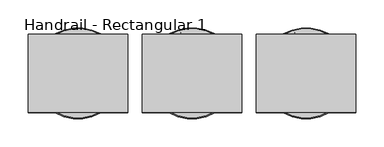
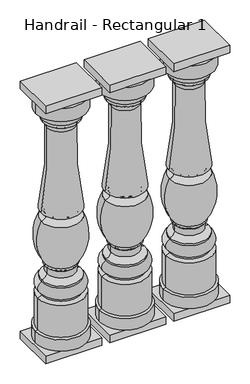
"""IFC4 building model written with IfcOpenShell, lengths in millimetres: railing geometry, Handrail - Rectangular 1."""

from ifc_helpers import new_model, si_unit, point, frame, origin, place, context, project, spatial, polyline, circle_curve, ellipse_curve, trimmed, outline, extrude, source, transform, mapped, element, save
from ifc_brep_helpers import plane_surface, cylinder_surface, revolved_surface, advanced_brep


def handrail_rectangular_1_f9308160(model_context):
    return source(origin(), model_context, "Body", "SolidModel", [
        advanced_brep(
        [(7223.6521895, -1665.6164768, 939.8), (7144.2771895, -1665.6164768, 939.8), (7303.0271895, -1665.6164768, 939.8), (7304.6146895, -1665.6164768, 127.0), (7142.6896895, -1665.6164768, 127.0), (7223.6521895, -1665.6164768, 127.0), (7304.6146895, -1665.6164768, 165.2785542), (7142.6896895, -1665.6164768, 165.2785542), (7297.4709395, -1665.6164768, 168.275), (7149.8334395, -1665.6164768, 168.275), (7297.4709395, -1665.6164768, 274.7335284), (7149.8334395, -1665.6164768, 274.7335284), (7284.7709395, -1665.6164768, 280.19375), (7162.5334395, -1665.6164768, 280.19375), (7284.7709395, -1665.6164768, 286.54375), (7162.5334395, -1665.6164768, 286.54375), (7284.7709395, -1665.6164768, 324.64375), (7162.5334395, -1665.6164768, 324.64375), (7284.7709395, -1665.6164768, 330.99375), (7162.5334395, -1665.6164768, 330.99375), (7269.0640435, -1665.6164768, 347.276159), (7178.2403356, -1665.6164768, 347.276159), (7269.0640435, -1665.6164768, 368.8906259), (7178.2403356, -1665.6164768, 368.8906259), (7273.6584395, -1665.6164768, 373.85625), (7173.6459395, -1665.6164768, 373.85625), (7273.6584395, -1665.6164768, 381.4842759), (7173.6459395, -1665.6164768, 381.4842759), (7286.3584395, -1665.6164768, 527.84375), (7160.9459395, -1665.6164768, 527.84375), (7286.3584395, -1665.6164768, 556.41875), (7160.9459395, -1665.6164768, 556.41875), (7267.8243377, -1665.6164768, 836.1713606), (7179.4800414, -1665.6164768, 836.1713606), (7280.8021895, -1665.6164768, 858.04375), (7166.5021895, -1665.6164768, 858.04375), (7280.8021895, -1665.6164768, 866.775), (7166.5021895, -1665.6164768, 866.775), (7291.9146895, -1665.6164768, 892.175), (7155.3896895, -1665.6164768, 892.175), (7303.0271895, -1665.6164768, 895.35), (7144.2771895, -1665.6164768, 895.35)],
        [
            (0, 1),
            (1, 2, circle_curve(frame((7223.6521895, -1665.6164768, 939.8), z_axis=(0.0, 0.0, 1.0), x_axis=(-1.0, 0.0, 0.0)), 79.375)),
            (2, 0),
            (2, 1, circle_curve(frame((7223.6521895, -1665.6164768, 939.8), z_axis=(0.0, 0.0, 1.0), x_axis=(-1.0, 0.0, 0.0)), 79.375)),
            (3, 4, circle_curve(frame((7223.6521895, -1665.6164768, 127.0), z_axis=(0.0, 0.0, -1.0), x_axis=(-1.0, 0.0, 0.0)), 80.9625)),
            (4, 5),
            (5, 3),
            (4, 3, circle_curve(frame((7223.6521895, -1665.6164768, 127.0), z_axis=(0.0, 0.0, -1.0), x_axis=(-1.0, 0.0, 0.0)), 80.9625)),
            (6, 7, circle_curve(frame((7223.6521895, -1665.6164768, 165.2785542), z_axis=(0.0, 0.0, -1.0), x_axis=(-1.0, 0.0, 0.0)), 80.9625)),
            (7, 4),
            (3, 6),
            (7, 6, circle_curve(frame((7223.6521895, -1665.6164768, 165.2785542), z_axis=(0.0, 0.0, -1.0), x_axis=(-1.0, 0.0, 0.0)), 80.9625)),
            (8, 9, circle_curve(frame((7223.6521895, -1665.6164768, 168.275), z_axis=(0.0, 0.0, -1.0), x_axis=(-1.0, 0.0, 0.0)), 73.81875)),
            (9, 7),
            (6, 8),
            (9, 8, circle_curve(frame((7223.6521895, -1665.6164768, 168.275), z_axis=(0.0, 0.0, -1.0), x_axis=(-1.0, 0.0, 0.0)), 73.81875)),
            (10, 11, circle_curve(frame((7223.6521895, -1665.6164768, 274.7335284), z_axis=(0.0, 0.0, -1.0), x_axis=(-1.0, 0.0, 0.0)), 73.81875)),
            (11, 9),
            (8, 10),
            (11, 10, circle_curve(frame((7223.6521895, -1665.6164768, 274.7335284), z_axis=(0.0, 0.0, -1.0), x_axis=(-1.0, 0.0, 0.0)), 73.81875)),
            (12, 13, circle_curve(frame((7223.6521895, -1665.6164768, 280.19375), z_axis=(0.0, 0.0, -1.0), x_axis=(-1.0, 0.0, 0.0)), 61.11875)),
            (13, 11),
            (10, 12),
            (13, 12, circle_curve(frame((7223.6521895, -1665.6164768, 280.19375), z_axis=(0.0, 0.0, -1.0), x_axis=(-1.0, 0.0, 0.0)), 61.11875)),
            (14, 15, circle_curve(frame((7223.6521895, -1665.6164768, 286.54375), z_axis=(0.0, 0.0, -1.0), x_axis=(-1.0, 0.0, 0.0)), 61.11875)),
            (15, 13),
            (12, 14),
            (15, 14, circle_curve(frame((7223.6521895, -1665.6164768, 286.54375), z_axis=(0.0, 0.0, -1.0), x_axis=(-1.0, 0.0, 0.0)), 61.11875)),
            (16, 17, circle_curve(frame((7223.6521895, -1665.6164768, 324.64375), z_axis=(0.0, 0.0, -1.0), x_axis=(-1.0, 0.0, 0.0)), 61.11875)),
            (17, 15, circle_curve(frame((7170.7987498, -1665.6164768, 305.59375), z_axis=(0.0, -1.0, 0.0), x_axis=(1.0, 0.0, 0.0)), 20.7657856)),
            (14, 16, circle_curve(frame((7276.5056293, -1665.6164768, 305.59375), z_axis=(0.0, -1.0, 0.0), x_axis=(-1.0, 0.0, 0.0)), 20.7657856)),
            (17, 16, circle_curve(frame((7223.6521895, -1665.6164768, 324.64375), z_axis=(0.0, 0.0, -1.0), x_axis=(-1.0, 0.0, 0.0)), 61.11875)),
            (18, 19, circle_curve(frame((7223.6521895, -1665.6164768, 330.99375), z_axis=(0.0, 0.0, -1.0), x_axis=(-1.0, 0.0, 0.0)), 61.11875)),
            (19, 17),
            (16, 18),
            (19, 18, circle_curve(frame((7223.6521895, -1665.6164768, 330.99375), z_axis=(0.0, 0.0, -1.0), x_axis=(-1.0, 0.0, 0.0)), 61.11875)),
            (20, 21, circle_curve(frame((7223.6521895, -1665.6164768, 347.276159), z_axis=(0.0, 0.0, -1.0), x_axis=(-1.0, 0.0, 0.0)), 45.4118539)),
            (21, 19, circle_curve(frame((7163.0004121, -1665.6164768, 346.26035), z_axis=(0.0, 1.0, 0.0), x_axis=(1.0, 0.0, 0.0)), 15.2737402)),
            (18, 20, circle_curve(frame((7284.303967, -1665.6164768, 346.26035), z_axis=(0.0, 1.0, 0.0), x_axis=(-1.0, 0.0, 0.0)), 15.2737402)),
            (21, 20, circle_curve(frame((7223.6521895, -1665.6164768, 347.276159), z_axis=(0.0, 0.0, -1.0), x_axis=(-1.0, 0.0, 0.0)), 45.4118539)),
            (22, 23, circle_curve(frame((7223.6521895, -1665.6164768, 368.8906259), z_axis=(0.0, 0.0, -1.0), x_axis=(-1.0, 0.0, 0.0)), 45.4118539)),
            (23, 21),
            (20, 22),
            (23, 22, circle_curve(frame((7223.6521895, -1665.6164768, 368.8906259), z_axis=(0.0, 0.0, -1.0), x_axis=(-1.0, 0.0, 0.0)), 45.4118539)),
            (24, 25, circle_curve(frame((7223.6521895, -1665.6164768, 373.85625), z_axis=(0.0, 0.0, -1.0), x_axis=(-1.0, 0.0, 0.0)), 50.00625)),
            (25, 23, circle_curve(frame((7173.3940931, -1665.6164768, 369.014959), z_axis=(0.0, 1.0, 0.0), x_axis=(1.0, 0.0, 0.0)), 4.8478372)),
            (22, 24, circle_curve(frame((7273.910286, -1665.6164768, 369.014959), z_axis=(0.0, 1.0, 0.0), x_axis=(-1.0, 0.0, 0.0)), 4.8478372)),
            (25, 24, circle_curve(frame((7223.6521895, -1665.6164768, 373.85625), z_axis=(0.0, 0.0, -1.0), x_axis=(-1.0, 0.0, 0.0)), 50.00625)),
            (26, 27, circle_curve(frame((7223.6521895, -1665.6164768, 381.4842759), z_axis=(0.0, 0.0, -1.0), x_axis=(-1.0, 0.0, 0.0)), 50.00625)),
            (27, 25),
            (24, 26),
            (27, 26, circle_curve(frame((7223.6521895, -1665.6164768, 381.4842759), z_axis=(0.0, 0.0, -1.0), x_axis=(-1.0, 0.0, 0.0)), 50.00625)),
            (28, 29, circle_curve(frame((7223.6521895, -1665.6164768, 527.84375), z_axis=(0.0, 0.0, -1.0), x_axis=(-1.0, 0.0, 0.0)), 62.70625)),
            (29, 27, circle_curve(frame((7291.2829206, -1665.6164768, 465.4226923), z_axis=(0.0, -1.0, 0.0), x_axis=(1.0, 0.0, 0.0)), 144.5133802)),
            (26, 28, circle_curve(frame((7156.0214585, -1665.6164768, 465.4226923), z_axis=(0.0, -1.0, 0.0), x_axis=(-1.0, 0.0, 0.0)), 144.5133802)),
            (29, 28, circle_curve(frame((7223.6521895, -1665.6164768, 527.84375), z_axis=(0.0, 0.0, -1.0), x_axis=(-1.0, 0.0, 0.0)), 62.70625)),
            (30, 31, circle_curve(frame((7223.6521895, -1665.6164768, 556.41875), z_axis=(0.0, 0.0, -1.0), x_axis=(-1.0, 0.0, 0.0)), 62.70625)),
            (31, 29, circle_curve(frame((7161.7940628, -1665.6164768, 542.13125), z_axis=(0.0, 1.0, 0.0), x_axis=(1.0, 0.0, 0.0)), 14.3126507)),
            (28, 30, circle_curve(frame((7285.5103163, -1665.6164768, 542.13125), z_axis=(0.0, 1.0, 0.0), x_axis=(-1.0, 0.0, 0.0)), 14.3126507)),
            (31, 30, circle_curve(frame((7223.6521895, -1665.6164768, 556.41875), z_axis=(0.0, 0.0, -1.0), x_axis=(-1.0, 0.0, 0.0)), 62.70625)),
            (32, 33, circle_curve(frame((7223.6521895, -1665.6164768, 836.1713606), z_axis=(0.0, 0.0, -1.0), x_axis=(-1.0, 0.0, 0.0)), 44.1721482)),
            (33, 31, circle_curve(frame((6049.660691, -1665.6164768, 770.5336134), z_axis=(0.0, 1.0, 0.0), x_axis=(1.0, 0.0, 0.0)), 1131.7243827)),
            (30, 32, circle_curve(frame((8397.6436881, -1665.6164768, 770.5336134), z_axis=(0.0, 1.0, 0.0), x_axis=(-1.0, 0.0, 0.0)), 1131.7243827)),
            (33, 32, circle_curve(frame((7223.6521895, -1665.6164768, 836.1713606), z_axis=(0.0, 0.0, -1.0), x_axis=(-1.0, 0.0, 0.0)), 44.1721482)),
            (34, 35, circle_curve(frame((7223.6521895, -1665.6164768, 858.04375), z_axis=(0.0, 0.0, -1.0), x_axis=(-1.0, 0.0, 0.0)), 57.15)),
            (35, 33, circle_curve(frame((7158.4577367, -1665.6164768, 838.4842616), z_axis=(0.0, 1.0, 0.0), x_axis=(1.0, 0.0, 0.0)), 21.1491562)),
            (32, 34, circle_curve(frame((7288.8466424, -1665.6164768, 838.4842616), z_axis=(0.0, 1.0, 0.0), x_axis=(-1.0, 0.0, 0.0)), 21.1491562)),
            (35, 34, circle_curve(frame((7223.6521895, -1665.6164768, 858.04375), z_axis=(0.0, 0.0, -1.0), x_axis=(-1.0, 0.0, 0.0)), 57.15)),
            (36, 37, circle_curve(frame((7223.6521895, -1665.6164768, 866.775), z_axis=(0.0, 0.0, -1.0), x_axis=(-1.0, 0.0, 0.0)), 57.15)),
            (37, 35),
            (34, 36),
            (37, 36, circle_curve(frame((7223.6521895, -1665.6164768, 866.775), z_axis=(0.0, 0.0, -1.0), x_axis=(-1.0, 0.0, 0.0)), 57.15)),
            (38, 39, circle_curve(frame((7223.6521895, -1665.6164768, 892.175), z_axis=(0.0, 0.0, -1.0), x_axis=(-1.0, 0.0, 0.0)), 68.2625)),
            (39, 37, circle_curve(frame((7184.7272944, -1665.6164768, 889.8793427), z_axis=(0.0, -1.0, 0.0), x_axis=(1.0, 0.0, 0.0)), 29.4272849)),
            (36, 38, circle_curve(frame((7262.5770847, -1665.6164768, 889.8793427), z_axis=(0.0, -1.0, 0.0), x_axis=(-1.0, 0.0, 0.0)), 29.4272849)),
            (39, 38, circle_curve(frame((7223.6521895, -1665.6164768, 892.175), z_axis=(0.0, 0.0, -1.0), x_axis=(-1.0, 0.0, 0.0)), 68.2625)),
            (40, 41, circle_curve(frame((7223.6521895, -1665.6164768, 895.35), z_axis=(0.0, 0.0, -1.0), x_axis=(-1.0, 0.0, 0.0)), 79.375)),
            (41, 39),
            (38, 40),
            (41, 40, circle_curve(frame((7223.6521895, -1665.6164768, 895.35), z_axis=(0.0, 0.0, -1.0), x_axis=(-1.0, 0.0, 0.0)), 79.375)),
            (1, 41),
            (40, 2),
        ],
        [
            plane_surface(frame((7223.6521895, -1665.6164768, 939.8), z_axis=(0.0, 0.0, 1.0), x_axis=(-1.0, 0.0, 0.0))),
            plane_surface(frame((7223.6521895, -1665.6164768, 127.0), z_axis=(0.0, 0.0, -1.0), x_axis=(-1.0, 0.0, 0.0))),
            cylinder_surface(frame((7223.6521895, -1665.6164768, 1009.65), z_axis=(0.0, 0.0, 1.0), x_axis=(-1.0, 0.0, 0.0)), 80.9625),
            revolved_surface(polyline([(7142.6896895, -1665.6164768, 165.2785542), (7149.8334395, -1665.6164768, 168.275)]), (7223.6521895, -1665.6164768, 1009.65), (0.0, 0.0, 1.0)),
            cylinder_surface(frame((7223.6521895, -1665.6164768, 1009.65), z_axis=(0.0, 0.0, 1.0), x_axis=(-1.0, 0.0, 0.0)), 73.81875),
            revolved_surface(polyline([(7149.8334395, -1665.6164768, 274.7335284), (7162.5334395, -1665.6164768, 280.19375)]), (7223.6521895, -1665.6164768, 1009.65), (0.0, 0.0, 1.0)),
            cylinder_surface(frame((7223.6521895, -1665.6164768, 1009.65), z_axis=(0.0, 0.0, 1.0), x_axis=(-1.0, 0.0, 0.0)), 61.11875),
            revolved_surface(trimmed(ellipse_curve(frame((7170.7987498, -1665.6164768, 305.59375), z_axis=(0.0, 1.0, 0.0), x_axis=(1.0, 0.0, 0.0)), 20.7657856, 20.7657856), [point((7162.5334395, -1665.6164768, 286.54375))], [point((7162.5334395, -1665.6164768, 324.64375))], True, "CARTESIAN"), (7223.6521895, -1665.6164768, 1009.65), (0.0, 0.0, 1.0)),
            revolved_surface(trimmed(ellipse_curve(frame((7163.0004121, -1665.6164768, 346.26035), z_axis=(0.0, -1.0, 0.0), x_axis=(1.0, 0.0, 0.0)), 15.2737402, 15.2737402), [point((7162.5334395, -1665.6164768, 330.99375))], [point((7178.2403356, -1665.6164768, 347.276159))], True, "CARTESIAN"), (7223.6521895, -1665.6164768, 1009.65), (0.0, 0.0, 1.0)),
            cylinder_surface(frame((7223.6521895, -1665.6164768, 1009.65), z_axis=(0.0, 0.0, 1.0), x_axis=(-1.0, 0.0, 0.0)), 45.4118539),
            revolved_surface(trimmed(ellipse_curve(frame((7173.3940931, -1665.6164768, 369.014959), z_axis=(0.0, -1.0, 0.0), x_axis=(1.0, 0.0, 0.0)), 4.8478372, 4.8478372), [point((7178.2403356, -1665.6164768, 368.8906259))], [point((7173.6459395, -1665.6164768, 373.85625))], True, "CARTESIAN"), (7223.6521895, -1665.6164768, 1009.65), (0.0, 0.0, 1.0)),
            cylinder_surface(frame((7223.6521895, -1665.6164768, 1009.65), z_axis=(0.0, 0.0, 1.0), x_axis=(-1.0, 0.0, 0.0)), 50.00625),
            revolved_surface(trimmed(ellipse_curve(frame((7291.2829206, -1665.6164768, 465.4226923), z_axis=(0.0, 1.0, 0.0), x_axis=(1.0, 0.0, 0.0)), 144.5133802, 144.5133802), [point((7173.6459395, -1665.6164768, 381.4842759))], [point((7160.9459395, -1665.6164768, 527.84375))], True, "CARTESIAN"), (7223.6521895, -1665.6164768, 1009.65), (0.0, 0.0, 1.0)),
            revolved_surface(trimmed(ellipse_curve(frame((7161.7940628, -1665.6164768, 542.13125), z_axis=(0.0, -1.0, 0.0), x_axis=(1.0, 0.0, 0.0)), 14.3126507, 14.3126507), [point((7160.9459395, -1665.6164768, 527.84375))], [point((7160.9459395, -1665.6164768, 556.41875))], True, "CARTESIAN"), (7223.6521895, -1665.6164768, 1009.65), (0.0, 0.0, 1.0)),
            revolved_surface(trimmed(ellipse_curve(frame((6049.660691, -1665.6164768, 770.5336134), z_axis=(0.0, -1.0, 0.0), x_axis=(1.0, 0.0, 0.0)), 1131.7243827, 1131.7243827), [point((7160.9459395, -1665.6164768, 556.41875))], [point((7179.4800414, -1665.6164768, 836.1713606))], True, "CARTESIAN"), (7223.6521895, -1665.6164768, 1009.65), (0.0, 0.0, 1.0)),
            revolved_surface(trimmed(ellipse_curve(frame((7158.4577367, -1665.6164768, 838.4842616), z_axis=(0.0, -1.0, 0.0), x_axis=(1.0, 0.0, 0.0)), 21.1491562, 21.1491562), [point((7179.4800414, -1665.6164768, 836.1713606))], [point((7166.5021895, -1665.6164768, 858.04375))], True, "CARTESIAN"), (7223.6521895, -1665.6164768, 1009.65), (0.0, 0.0, 1.0)),
            cylinder_surface(frame((7223.6521895, -1665.6164768, 1009.65), z_axis=(0.0, 0.0, 1.0), x_axis=(-1.0, 0.0, 0.0)), 57.15),
            revolved_surface(trimmed(ellipse_curve(frame((7184.7272944, -1665.6164768, 889.8793427), z_axis=(0.0, 1.0, 0.0), x_axis=(1.0, 0.0, 0.0)), 29.4272849, 29.4272849), [point((7166.5021895, -1665.6164768, 866.775))], [point((7155.3896895, -1665.6164768, 892.175))], True, "CARTESIAN"), (7223.6521895, -1665.6164768, 1009.65), (0.0, 0.0, 1.0)),
            revolved_surface(polyline([(7155.3896895, -1665.6164768, 892.175), (7144.2771895, -1665.6164768, 895.35)]), (7223.6521895, -1665.6164768, 1009.65), (0.0, 0.0, 1.0)),
            cylinder_surface(frame((7223.6521895, -1665.6164768, 1009.65), z_axis=(0.0, 0.0, 1.0), x_axis=(-1.0, 0.0, 0.0)), 79.375),
        ],
        [
            (0, [[1, 2, 3]]),
            (0, [[-3, 4, -1]]),
            (1, [[5, 6, 7]]),
            (1, [[8, -7, -6]]),
            (2, [[9, 10, -5, 11]]),
            (2, [[12, -11, -8, -10]]),
            (3, [[13, 14, -9, 15]]),
            (3, [[16, -15, -12, -14]]),
            (4, [[17, 18, -13, 19]]),
            (4, [[20, -19, -16, -18]]),
            (5, [[21, 22, -17, 23]]),
            (5, [[24, -23, -20, -22]]),
            (6, [[25, 26, -21, 27]]),
            (6, [[28, -27, -24, -26]]),
            (7, [[29, 30, -25, 31]]),
            (7, [[32, -31, -28, -30]]),
            (6, [[33, 34, -29, 35]]),
            (6, [[36, -35, -32, -34]]),
            (8, [[37, 38, -33, 39]]),
            (8, [[40, -39, -36, -38]]),
            (9, [[41, 42, -37, 43]]),
            (9, [[44, -43, -40, -42]]),
            (10, [[45, 46, -41, 47]]),
            (10, [[48, -47, -44, -46]]),
            (11, [[49, 50, -45, 51]]),
            (11, [[52, -51, -48, -50]]),
            (12, [[53, 54, -49, 55]]),
            (12, [[56, -55, -52, -54]]),
            (13, [[57, 58, -53, 59]]),
            (13, [[60, -59, -56, -58]]),
            (14, [[61, 62, -57, 63]]),
            (14, [[64, -63, -60, -62]]),
            (15, [[65, 66, -61, 67]]),
            (15, [[68, -67, -64, -66]]),
            (16, [[69, 70, -65, 71]]),
            (16, [[72, -71, -68, -70]]),
            (17, [[73, 74, -69, 75]]),
            (17, [[76, -75, -72, -74]]),
            (18, [[77, 78, -73, 79]]),
            (18, [[80, -79, -76, -78]]),
            (19, [[-2, 81, -77, 82]]),
            (19, [[-4, -82, -80, -81]]),
        ],
    ),
        extrude(outline(polyline([(7134.7521895, -1735.4664768), (7134.7521895, -1595.7664768), (7312.5521895, -1595.7664768), (7312.5521895, -1735.4664768), (7134.7521895, -1735.4664768)])), frame((0.0, 0.0, 101.6), z_axis=(0.0, 0.0, 1.0), x_axis=(1.0, 0.0, 0.0)), (0.0, 0.0, 1.0), 25.4),
        extrude(outline(polyline([(7134.7521895, -1595.7664768), (7312.5521895, -1595.7664768), (7312.5521895, -1735.4664768), (7134.7521895, -1735.4664768), (7134.7521895, -1595.7664768)])), frame((0.0, 0.0, 939.8), z_axis=(0.0, 0.0, 1.0), x_axis=(1.0, 0.0, 0.0)), (0.0, 0.0, 1.0), 25.4),
        advanced_brep(
        [(7020.4521895, -1665.6164768, 939.8), (6941.0771895, -1665.6164768, 939.8), (7099.8271895, -1665.6164768, 939.8), (7101.4146895, -1665.6164768, 127.0), (6939.4896895, -1665.6164768, 127.0), (7020.4521895, -1665.6164768, 127.0), (7101.4146895, -1665.6164768, 165.2785542), (6939.4896895, -1665.6164768, 165.2785542), (7094.2709395, -1665.6164768, 168.275), (6946.6334395, -1665.6164768, 168.275), (7094.2709395, -1665.6164768, 274.7335284), (6946.6334395, -1665.6164768, 274.7335284), (7081.5709395, -1665.6164768, 280.19375), (6959.3334395, -1665.6164768, 280.19375), (7081.5709395, -1665.6164768, 286.54375), (6959.3334395, -1665.6164768, 286.54375), (7081.5709395, -1665.6164768, 324.64375), (6959.3334395, -1665.6164768, 324.64375), (7081.5709395, -1665.6164768, 330.99375), (6959.3334395, -1665.6164768, 330.99375), (7065.8640435, -1665.6164768, 347.276159), (6975.0403356, -1665.6164768, 347.276159), (7065.8640435, -1665.6164768, 368.8906259), (6975.0403356, -1665.6164768, 368.8906259), (7070.4584395, -1665.6164768, 373.85625), (6970.4459395, -1665.6164768, 373.85625), (7070.4584395, -1665.6164768, 381.4842759), (6970.4459395, -1665.6164768, 381.4842759), (7083.1584395, -1665.6164768, 527.84375), (6957.7459395, -1665.6164768, 527.84375), (7083.1584395, -1665.6164768, 556.41875), (6957.7459395, -1665.6164768, 556.41875), (7064.6243377, -1665.6164768, 836.1713606), (6976.2800414, -1665.6164768, 836.1713606), (7077.6021895, -1665.6164768, 858.04375), (6963.3021895, -1665.6164768, 858.04375), (7077.6021895, -1665.6164768, 866.775), (6963.3021895, -1665.6164768, 866.775), (7088.7146895, -1665.6164768, 892.175), (6952.1896895, -1665.6164768, 892.175), (7099.8271895, -1665.6164768, 895.35), (6941.0771895, -1665.6164768, 895.35)],
        [
            (0, 1),
            (1, 2, circle_curve(frame((7020.4521895, -1665.6164768, 939.8), z_axis=(0.0, 0.0, 1.0), x_axis=(-1.0, 0.0, 0.0)), 79.375)),
            (2, 0),
            (2, 1, circle_curve(frame((7020.4521895, -1665.6164768, 939.8), z_axis=(0.0, 0.0, 1.0), x_axis=(-1.0, 0.0, 0.0)), 79.375)),
            (3, 4, circle_curve(frame((7020.4521895, -1665.6164768, 127.0), z_axis=(0.0, 0.0, -1.0), x_axis=(-1.0, 0.0, 0.0)), 80.9625)),
            (4, 5),
            (5, 3),
            (4, 3, circle_curve(frame((7020.4521895, -1665.6164768, 127.0), z_axis=(0.0, 0.0, -1.0), x_axis=(-1.0, 0.0, 0.0)), 80.9625)),
            (6, 7, circle_curve(frame((7020.4521895, -1665.6164768, 165.2785542), z_axis=(0.0, 0.0, -1.0), x_axis=(-1.0, 0.0, 0.0)), 80.9625)),
            (7, 4),
            (3, 6),
            (7, 6, circle_curve(frame((7020.4521895, -1665.6164768, 165.2785542), z_axis=(0.0, 0.0, -1.0), x_axis=(-1.0, 0.0, 0.0)), 80.9625)),
            (8, 9, circle_curve(frame((7020.4521895, -1665.6164768, 168.275), z_axis=(0.0, 0.0, -1.0), x_axis=(-1.0, 0.0, 0.0)), 73.81875)),
            (9, 7),
            (6, 8),
            (9, 8, circle_curve(frame((7020.4521895, -1665.6164768, 168.275), z_axis=(0.0, 0.0, -1.0), x_axis=(-1.0, 0.0, 0.0)), 73.81875)),
            (10, 11, circle_curve(frame((7020.4521895, -1665.6164768, 274.7335284), z_axis=(0.0, 0.0, -1.0), x_axis=(-1.0, 0.0, 0.0)), 73.81875)),
            (11, 9),
            (8, 10),
            (11, 10, circle_curve(frame((7020.4521895, -1665.6164768, 274.7335284), z_axis=(0.0, 0.0, -1.0), x_axis=(-1.0, 0.0, 0.0)), 73.81875)),
            (12, 13, circle_curve(frame((7020.4521895, -1665.6164768, 280.19375), z_axis=(0.0, 0.0, -1.0), x_axis=(-1.0, 0.0, 0.0)), 61.11875)),
            (13, 11),
            (10, 12),
            (13, 12, circle_curve(frame((7020.4521895, -1665.6164768, 280.19375), z_axis=(0.0, 0.0, -1.0), x_axis=(-1.0, 0.0, 0.0)), 61.11875)),
            (14, 15, circle_curve(frame((7020.4521895, -1665.6164768, 286.54375), z_axis=(0.0, 0.0, -1.0), x_axis=(-1.0, 0.0, 0.0)), 61.11875)),
            (15, 13),
            (12, 14),
            (15, 14, circle_curve(frame((7020.4521895, -1665.6164768, 286.54375), z_axis=(0.0, 0.0, -1.0), x_axis=(-1.0, 0.0, 0.0)), 61.11875)),
            (16, 17, circle_curve(frame((7020.4521895, -1665.6164768, 324.64375), z_axis=(0.0, 0.0, -1.0), x_axis=(-1.0, 0.0, 0.0)), 61.11875)),
            (17, 15, circle_curve(frame((6967.5987498, -1665.6164768, 305.59375), z_axis=(0.0, -1.0, 0.0), x_axis=(1.0, 0.0, 0.0)), 20.7657856)),
            (14, 16, circle_curve(frame((7073.3056293, -1665.6164768, 305.59375), z_axis=(0.0, -1.0, 0.0), x_axis=(-1.0, 0.0, 0.0)), 20.7657856)),
            (17, 16, circle_curve(frame((7020.4521895, -1665.6164768, 324.64375), z_axis=(0.0, 0.0, -1.0), x_axis=(-1.0, 0.0, 0.0)), 61.11875)),
            (18, 19, circle_curve(frame((7020.4521895, -1665.6164768, 330.99375), z_axis=(0.0, 0.0, -1.0), x_axis=(-1.0, 0.0, 0.0)), 61.11875)),
            (19, 17),
            (16, 18),
            (19, 18, circle_curve(frame((7020.4521895, -1665.6164768, 330.99375), z_axis=(0.0, 0.0, -1.0), x_axis=(-1.0, 0.0, 0.0)), 61.11875)),
            (20, 21, circle_curve(frame((7020.4521895, -1665.6164768, 347.276159), z_axis=(0.0, 0.0, -1.0), x_axis=(-1.0, 0.0, 0.0)), 45.4118539)),
            (21, 19, circle_curve(frame((6959.8004121, -1665.6164768, 346.26035), z_axis=(0.0, 1.0, 0.0), x_axis=(1.0, 0.0, 0.0)), 15.2737402)),
            (18, 20, circle_curve(frame((7081.103967, -1665.6164768, 346.26035), z_axis=(0.0, 1.0, 0.0), x_axis=(-1.0, 0.0, 0.0)), 15.2737402)),
            (21, 20, circle_curve(frame((7020.4521895, -1665.6164768, 347.276159), z_axis=(0.0, 0.0, -1.0), x_axis=(-1.0, 0.0, 0.0)), 45.4118539)),
            (22, 23, circle_curve(frame((7020.4521895, -1665.6164768, 368.8906259), z_axis=(0.0, 0.0, -1.0), x_axis=(-1.0, 0.0, 0.0)), 45.4118539)),
            (23, 21),
            (20, 22),
            (23, 22, circle_curve(frame((7020.4521895, -1665.6164768, 368.8906259), z_axis=(0.0, 0.0, -1.0), x_axis=(-1.0, 0.0, 0.0)), 45.4118539)),
            (24, 25, circle_curve(frame((7020.4521895, -1665.6164768, 373.85625), z_axis=(0.0, 0.0, -1.0), x_axis=(-1.0, 0.0, 0.0)), 50.00625)),
            (25, 23, circle_curve(frame((6970.1940931, -1665.6164768, 369.014959), z_axis=(0.0, 1.0, 0.0), x_axis=(1.0, 0.0, 0.0)), 4.8478372)),
            (22, 24, circle_curve(frame((7070.710286, -1665.6164768, 369.014959), z_axis=(0.0, 1.0, 0.0), x_axis=(-1.0, 0.0, 0.0)), 4.8478372)),
            (25, 24, circle_curve(frame((7020.4521895, -1665.6164768, 373.85625), z_axis=(0.0, 0.0, -1.0), x_axis=(-1.0, 0.0, 0.0)), 50.00625)),
            (26, 27, circle_curve(frame((7020.4521895, -1665.6164768, 381.4842759), z_axis=(0.0, 0.0, -1.0), x_axis=(-1.0, 0.0, 0.0)), 50.00625)),
            (27, 25),
            (24, 26),
            (27, 26, circle_curve(frame((7020.4521895, -1665.6164768, 381.4842759), z_axis=(0.0, 0.0, -1.0), x_axis=(-1.0, 0.0, 0.0)), 50.00625)),
            (28, 29, circle_curve(frame((7020.4521895, -1665.6164768, 527.84375), z_axis=(0.0, 0.0, -1.0), x_axis=(-1.0, 0.0, 0.0)), 62.70625)),
            (29, 27, circle_curve(frame((7088.0829206, -1665.6164768, 465.4226923), z_axis=(0.0, -1.0, 0.0), x_axis=(1.0, 0.0, 0.0)), 144.5133802)),
            (26, 28, circle_curve(frame((6952.8214585, -1665.6164768, 465.4226923), z_axis=(0.0, -1.0, 0.0), x_axis=(-1.0, 0.0, 0.0)), 144.5133802)),
            (29, 28, circle_curve(frame((7020.4521895, -1665.6164768, 527.84375), z_axis=(0.0, 0.0, -1.0), x_axis=(-1.0, 0.0, 0.0)), 62.70625)),
            (30, 31, circle_curve(frame((7020.4521895, -1665.6164768, 556.41875), z_axis=(0.0, 0.0, -1.0), x_axis=(-1.0, 0.0, 0.0)), 62.70625)),
            (31, 29, circle_curve(frame((6958.5940628, -1665.6164768, 542.13125), z_axis=(0.0, 1.0, 0.0), x_axis=(1.0, 0.0, 0.0)), 14.3126507)),
            (28, 30, circle_curve(frame((7082.3103163, -1665.6164768, 542.13125), z_axis=(0.0, 1.0, 0.0), x_axis=(-1.0, 0.0, 0.0)), 14.3126507)),
            (31, 30, circle_curve(frame((7020.4521895, -1665.6164768, 556.41875), z_axis=(0.0, 0.0, -1.0), x_axis=(-1.0, 0.0, 0.0)), 62.70625)),
            (32, 33, circle_curve(frame((7020.4521895, -1665.6164768, 836.1713606), z_axis=(0.0, 0.0, -1.0), x_axis=(-1.0, 0.0, 0.0)), 44.1721482)),
            (33, 31, circle_curve(frame((5846.460691, -1665.6164768, 770.5336134), z_axis=(0.0, 1.0, 0.0), x_axis=(1.0, 0.0, 0.0)), 1131.7243827)),
            (30, 32, circle_curve(frame((8194.4436881, -1665.6164768, 770.5336134), z_axis=(0.0, 1.0, 0.0), x_axis=(-1.0, 0.0, 0.0)), 1131.7243827)),
            (33, 32, circle_curve(frame((7020.4521895, -1665.6164768, 836.1713606), z_axis=(0.0, 0.0, -1.0), x_axis=(-1.0, 0.0, 0.0)), 44.1721482)),
            (34, 35, circle_curve(frame((7020.4521895, -1665.6164768, 858.04375), z_axis=(0.0, 0.0, -1.0), x_axis=(-1.0, 0.0, 0.0)), 57.15)),
            (35, 33, circle_curve(frame((6955.2577367, -1665.6164768, 838.4842616), z_axis=(0.0, 1.0, 0.0), x_axis=(1.0, 0.0, 0.0)), 21.1491562)),
            (32, 34, circle_curve(frame((7085.6466424, -1665.6164768, 838.4842616), z_axis=(0.0, 1.0, 0.0), x_axis=(-1.0, 0.0, 0.0)), 21.1491562)),
            (35, 34, circle_curve(frame((7020.4521895, -1665.6164768, 858.04375), z_axis=(0.0, 0.0, -1.0), x_axis=(-1.0, 0.0, 0.0)), 57.15)),
            (36, 37, circle_curve(frame((7020.4521895, -1665.6164768, 866.775), z_axis=(0.0, 0.0, -1.0), x_axis=(-1.0, 0.0, 0.0)), 57.15)),
            (37, 35),
            (34, 36),
            (37, 36, circle_curve(frame((7020.4521895, -1665.6164768, 866.775), z_axis=(0.0, 0.0, -1.0), x_axis=(-1.0, 0.0, 0.0)), 57.15)),
            (38, 39, circle_curve(frame((7020.4521895, -1665.6164768, 892.175), z_axis=(0.0, 0.0, -1.0), x_axis=(-1.0, 0.0, 0.0)), 68.2625)),
            (39, 37, circle_curve(frame((6981.5272944, -1665.6164768, 889.8793427), z_axis=(0.0, -1.0, 0.0), x_axis=(1.0, 0.0, 0.0)), 29.4272849)),
            (36, 38, circle_curve(frame((7059.3770847, -1665.6164768, 889.8793427), z_axis=(0.0, -1.0, 0.0), x_axis=(-1.0, 0.0, 0.0)), 29.4272849)),
            (39, 38, circle_curve(frame((7020.4521895, -1665.6164768, 892.175), z_axis=(0.0, 0.0, -1.0), x_axis=(-1.0, 0.0, 0.0)), 68.2625)),
            (40, 41, circle_curve(frame((7020.4521895, -1665.6164768, 895.35), z_axis=(0.0, 0.0, -1.0), x_axis=(-1.0, 0.0, 0.0)), 79.375)),
            (41, 39),
            (38, 40),
            (41, 40, circle_curve(frame((7020.4521895, -1665.6164768, 895.35), z_axis=(0.0, 0.0, -1.0), x_axis=(-1.0, 0.0, 0.0)), 79.375)),
            (1, 41),
            (40, 2),
        ],
        [
            plane_surface(frame((7020.4521895, -1665.6164768, 939.8), z_axis=(0.0, 0.0, 1.0), x_axis=(-1.0, 0.0, 0.0))),
            plane_surface(frame((7020.4521895, -1665.6164768, 127.0), z_axis=(0.0, 0.0, -1.0), x_axis=(-1.0, 0.0, 0.0))),
            cylinder_surface(frame((7020.4521895, -1665.6164768, 1009.65), z_axis=(0.0, 0.0, 1.0), x_axis=(-1.0, 0.0, 0.0)), 80.9625),
            revolved_surface(polyline([(6939.4896895, -1665.6164768, 165.2785542), (6946.6334395, -1665.6164768, 168.275)]), (7020.4521895, -1665.6164768, 1009.65), (0.0, 0.0, 1.0)),
            cylinder_surface(frame((7020.4521895, -1665.6164768, 1009.65), z_axis=(0.0, 0.0, 1.0), x_axis=(-1.0, 0.0, 0.0)), 73.81875),
            revolved_surface(polyline([(6946.6334395, -1665.6164768, 274.7335284), (6959.3334395, -1665.6164768, 280.19375)]), (7020.4521895, -1665.6164768, 1009.65), (0.0, 0.0, 1.0)),
            cylinder_surface(frame((7020.4521895, -1665.6164768, 1009.65), z_axis=(0.0, 0.0, 1.0), x_axis=(-1.0, 0.0, 0.0)), 61.11875),
            revolved_surface(trimmed(ellipse_curve(frame((6967.5987498, -1665.6164768, 305.59375), z_axis=(0.0, 1.0, 0.0), x_axis=(1.0, 0.0, 0.0)), 20.7657856, 20.7657856), [point((6959.3334395, -1665.6164768, 286.54375))], [point((6959.3334395, -1665.6164768, 324.64375))], True, "CARTESIAN"), (7020.4521895, -1665.6164768, 1009.65), (0.0, 0.0, 1.0)),
            revolved_surface(trimmed(ellipse_curve(frame((6959.8004121, -1665.6164768, 346.26035), z_axis=(0.0, -1.0, 0.0), x_axis=(1.0, 0.0, 0.0)), 15.2737402, 15.2737402), [point((6959.3334395, -1665.6164768, 330.99375))], [point((6975.0403356, -1665.6164768, 347.276159))], True, "CARTESIAN"), (7020.4521895, -1665.6164768, 1009.65), (0.0, 0.0, 1.0)),
            cylinder_surface(frame((7020.4521895, -1665.6164768, 1009.65), z_axis=(0.0, 0.0, 1.0), x_axis=(-1.0, 0.0, 0.0)), 45.4118539),
            revolved_surface(trimmed(ellipse_curve(frame((6970.1940931, -1665.6164768, 369.014959), z_axis=(0.0, -1.0, 0.0), x_axis=(1.0, 0.0, 0.0)), 4.8478372, 4.8478372), [point((6975.0403356, -1665.6164768, 368.8906259))], [point((6970.4459395, -1665.6164768, 373.85625))], True, "CARTESIAN"), (7020.4521895, -1665.6164768, 1009.65), (0.0, 0.0, 1.0)),
            cylinder_surface(frame((7020.4521895, -1665.6164768, 1009.65), z_axis=(0.0, 0.0, 1.0), x_axis=(-1.0, 0.0, 0.0)), 50.00625),
            revolved_surface(trimmed(ellipse_curve(frame((7088.0829206, -1665.6164768, 465.4226923), z_axis=(0.0, 1.0, 0.0), x_axis=(1.0, 0.0, 0.0)), 144.5133802, 144.5133802), [point((6970.4459395, -1665.6164768, 381.4842759))], [point((6957.7459395, -1665.6164768, 527.84375))], True, "CARTESIAN"), (7020.4521895, -1665.6164768, 1009.65), (0.0, 0.0, 1.0)),
            revolved_surface(trimmed(ellipse_curve(frame((6958.5940628, -1665.6164768, 542.13125), z_axis=(0.0, -1.0, 0.0), x_axis=(1.0, 0.0, 0.0)), 14.3126507, 14.3126507), [point((6957.7459395, -1665.6164768, 527.84375))], [point((6957.7459395, -1665.6164768, 556.41875))], True, "CARTESIAN"), (7020.4521895, -1665.6164768, 1009.65), (0.0, 0.0, 1.0)),
            revolved_surface(trimmed(ellipse_curve(frame((5846.460691, -1665.6164768, 770.5336134), z_axis=(0.0, -1.0, 0.0), x_axis=(1.0, 0.0, 0.0)), 1131.7243827, 1131.7243827), [point((6957.7459395, -1665.6164768, 556.41875))], [point((6976.2800414, -1665.6164768, 836.1713606))], True, "CARTESIAN"), (7020.4521895, -1665.6164768, 1009.65), (0.0, 0.0, 1.0)),
            revolved_surface(trimmed(ellipse_curve(frame((6955.2577367, -1665.6164768, 838.4842616), z_axis=(0.0, -1.0, 0.0), x_axis=(1.0, 0.0, 0.0)), 21.1491562, 21.1491562), [point((6976.2800414, -1665.6164768, 836.1713606))], [point((6963.3021895, -1665.6164768, 858.04375))], True, "CARTESIAN"), (7020.4521895, -1665.6164768, 1009.65), (0.0, 0.0, 1.0)),
            cylinder_surface(frame((7020.4521895, -1665.6164768, 1009.65), z_axis=(0.0, 0.0, 1.0), x_axis=(-1.0, 0.0, 0.0)), 57.15),
            revolved_surface(trimmed(ellipse_curve(frame((6981.5272944, -1665.6164768, 889.8793427), z_axis=(0.0, 1.0, 0.0), x_axis=(1.0, 0.0, 0.0)), 29.4272849, 29.4272849), [point((6963.3021895, -1665.6164768, 866.775))], [point((6952.1896895, -1665.6164768, 892.175))], True, "CARTESIAN"), (7020.4521895, -1665.6164768, 1009.65), (0.0, 0.0, 1.0)),
            revolved_surface(polyline([(6952.1896895, -1665.6164768, 892.175), (6941.0771895, -1665.6164768, 895.35)]), (7020.4521895, -1665.6164768, 1009.65), (0.0, 0.0, 1.0)),
            cylinder_surface(frame((7020.4521895, -1665.6164768, 1009.65), z_axis=(0.0, 0.0, 1.0), x_axis=(-1.0, 0.0, 0.0)), 79.375),
        ],
        [
            (0, [[1, 2, 3]]),
            (0, [[-3, 4, -1]]),
            (1, [[5, 6, 7]]),
            (1, [[8, -7, -6]]),
            (2, [[9, 10, -5, 11]]),
            (2, [[12, -11, -8, -10]]),
            (3, [[13, 14, -9, 15]]),
            (3, [[16, -15, -12, -14]]),
            (4, [[17, 18, -13, 19]]),
            (4, [[20, -19, -16, -18]]),
            (5, [[21, 22, -17, 23]]),
            (5, [[24, -23, -20, -22]]),
            (6, [[25, 26, -21, 27]]),
            (6, [[28, -27, -24, -26]]),
            (7, [[29, 30, -25, 31]]),
            (7, [[32, -31, -28, -30]]),
            (6, [[33, 34, -29, 35]]),
            (6, [[36, -35, -32, -34]]),
            (8, [[37, 38, -33, 39]]),
            (8, [[40, -39, -36, -38]]),
            (9, [[41, 42, -37, 43]]),
            (9, [[44, -43, -40, -42]]),
            (10, [[45, 46, -41, 47]]),
            (10, [[48, -47, -44, -46]]),
            (11, [[49, 50, -45, 51]]),
            (11, [[52, -51, -48, -50]]),
            (12, [[53, 54, -49, 55]]),
            (12, [[56, -55, -52, -54]]),
            (13, [[57, 58, -53, 59]]),
            (13, [[60, -59, -56, -58]]),
            (14, [[61, 62, -57, 63]]),
            (14, [[64, -63, -60, -62]]),
            (15, [[65, 66, -61, 67]]),
            (15, [[68, -67, -64, -66]]),
            (16, [[69, 70, -65, 71]]),
            (16, [[72, -71, -68, -70]]),
            (17, [[73, 74, -69, 75]]),
            (17, [[76, -75, -72, -74]]),
            (18, [[77, 78, -73, 79]]),
            (18, [[80, -79, -76, -78]]),
            (19, [[-2, 81, -77, 82]]),
            (19, [[-4, -82, -80, -81]]),
        ],
    ),
        extrude(outline(polyline([(6931.5521895, -1735.4664768), (6931.5521895, -1595.7664768), (7109.3521895, -1595.7664768), (7109.3521895, -1735.4664768), (6931.5521895, -1735.4664768)])), frame((0.0, 0.0, 101.6), z_axis=(0.0, 0.0, 1.0), x_axis=(1.0, 0.0, 0.0)), (0.0, 0.0, 1.0), 25.4),
        extrude(outline(polyline([(6931.5521895, -1595.7664768), (7109.3521895, -1595.7664768), (7109.3521895, -1735.4664768), (6931.5521895, -1735.4664768), (6931.5521895, -1595.7664768)])), frame((0.0, 0.0, 939.8), z_axis=(0.0, 0.0, 1.0), x_axis=(1.0, 0.0, 0.0)), (0.0, 0.0, 1.0), 25.4),
        advanced_brep(
        [(6817.2521895, -1665.6164768, 939.8), (6737.8771895, -1665.6164768, 939.8), (6896.6271895, -1665.6164768, 939.8), (6898.2146895, -1665.6164768, 127.0), (6736.2896895, -1665.6164768, 127.0), (6817.2521895, -1665.6164768, 127.0), (6898.2146895, -1665.6164768, 165.2785542), (6736.2896895, -1665.6164768, 165.2785542), (6891.0709395, -1665.6164768, 168.275), (6743.4334395, -1665.6164768, 168.275), (6891.0709395, -1665.6164768, 274.7335284), (6743.4334395, -1665.6164768, 274.7335284), (6878.3709395, -1665.6164768, 280.19375), (6756.1334395, -1665.6164768, 280.19375), (6878.3709395, -1665.6164768, 286.54375), (6756.1334395, -1665.6164768, 286.54375), (6878.3709395, -1665.6164768, 324.64375), (6756.1334395, -1665.6164768, 324.64375), (6878.3709395, -1665.6164768, 330.99375), (6756.1334395, -1665.6164768, 330.99375), (6862.6640435, -1665.6164768, 347.276159), (6771.8403356, -1665.6164768, 347.276159), (6862.6640435, -1665.6164768, 368.8906259), (6771.8403356, -1665.6164768, 368.8906259), (6867.2584395, -1665.6164768, 373.85625), (6767.2459395, -1665.6164768, 373.85625), (6867.2584395, -1665.6164768, 381.4842759), (6767.2459395, -1665.6164768, 381.4842759), (6879.9584395, -1665.6164768, 527.84375), (6754.5459395, -1665.6164768, 527.84375), (6879.9584395, -1665.6164768, 556.41875), (6754.5459395, -1665.6164768, 556.41875), (6861.4243377, -1665.6164768, 836.1713606), (6773.0800414, -1665.6164768, 836.1713606), (6874.4021895, -1665.6164768, 858.04375), (6760.1021895, -1665.6164768, 858.04375), (6874.4021895, -1665.6164768, 866.775), (6760.1021895, -1665.6164768, 866.775), (6885.5146895, -1665.6164768, 892.175), (6748.9896895, -1665.6164768, 892.175), (6896.6271895, -1665.6164768, 895.35), (6737.8771895, -1665.6164768, 895.35)],
        [
            (0, 1),
            (1, 2, circle_curve(frame((6817.2521895, -1665.6164768, 939.8), z_axis=(0.0, 0.0, 1.0), x_axis=(-1.0, 0.0, 0.0)), 79.375)),
            (2, 0),
            (2, 1, circle_curve(frame((6817.2521895, -1665.6164768, 939.8), z_axis=(0.0, 0.0, 1.0), x_axis=(-1.0, 0.0, 0.0)), 79.375)),
            (3, 4, circle_curve(frame((6817.2521895, -1665.6164768, 127.0), z_axis=(0.0, 0.0, -1.0), x_axis=(-1.0, 0.0, 0.0)), 80.9625)),
            (4, 5),
            (5, 3),
            (4, 3, circle_curve(frame((6817.2521895, -1665.6164768, 127.0), z_axis=(0.0, 0.0, -1.0), x_axis=(-1.0, 0.0, 0.0)), 80.9625)),
            (6, 7, circle_curve(frame((6817.2521895, -1665.6164768, 165.2785542), z_axis=(0.0, 0.0, -1.0), x_axis=(-1.0, 0.0, 0.0)), 80.9625)),
            (7, 4),
            (3, 6),
            (7, 6, circle_curve(frame((6817.2521895, -1665.6164768, 165.2785542), z_axis=(0.0, 0.0, -1.0), x_axis=(-1.0, 0.0, 0.0)), 80.9625)),
            (8, 9, circle_curve(frame((6817.2521895, -1665.6164768, 168.275), z_axis=(0.0, 0.0, -1.0), x_axis=(-1.0, 0.0, 0.0)), 73.81875)),
            (9, 7),
            (6, 8),
            (9, 8, circle_curve(frame((6817.2521895, -1665.6164768, 168.275), z_axis=(0.0, 0.0, -1.0), x_axis=(-1.0, 0.0, 0.0)), 73.81875)),
            (10, 11, circle_curve(frame((6817.2521895, -1665.6164768, 274.7335284), z_axis=(0.0, 0.0, -1.0), x_axis=(-1.0, 0.0, 0.0)), 73.81875)),
            (11, 9),
            (8, 10),
            (11, 10, circle_curve(frame((6817.2521895, -1665.6164768, 274.7335284), z_axis=(0.0, 0.0, -1.0), x_axis=(-1.0, 0.0, 0.0)), 73.81875)),
            (12, 13, circle_curve(frame((6817.2521895, -1665.6164768, 280.19375), z_axis=(0.0, 0.0, -1.0), x_axis=(-1.0, 0.0, 0.0)), 61.11875)),
            (13, 11),
            (10, 12),
            (13, 12, circle_curve(frame((6817.2521895, -1665.6164768, 280.19375), z_axis=(0.0, 0.0, -1.0), x_axis=(-1.0, 0.0, 0.0)), 61.11875)),
            (14, 15, circle_curve(frame((6817.2521895, -1665.6164768, 286.54375), z_axis=(0.0, 0.0, -1.0), x_axis=(-1.0, 0.0, 0.0)), 61.11875)),
            (15, 13),
            (12, 14),
            (15, 14, circle_curve(frame((6817.2521895, -1665.6164768, 286.54375), z_axis=(0.0, 0.0, -1.0), x_axis=(-1.0, 0.0, 0.0)), 61.11875)),
            (16, 17, circle_curve(frame((6817.2521895, -1665.6164768, 324.64375), z_axis=(0.0, 0.0, -1.0), x_axis=(-1.0, 0.0, 0.0)), 61.11875)),
            (17, 15, circle_curve(frame((6764.3987498, -1665.6164768, 305.59375), z_axis=(0.0, -1.0, 0.0), x_axis=(1.0, 0.0, 0.0)), 20.7657856)),
            (14, 16, circle_curve(frame((6870.1056293, -1665.6164768, 305.59375), z_axis=(0.0, -1.0, 0.0), x_axis=(-1.0, 0.0, 0.0)), 20.7657856)),
            (17, 16, circle_curve(frame((6817.2521895, -1665.6164768, 324.64375), z_axis=(0.0, 0.0, -1.0), x_axis=(-1.0, 0.0, 0.0)), 61.11875)),
            (18, 19, circle_curve(frame((6817.2521895, -1665.6164768, 330.99375), z_axis=(0.0, 0.0, -1.0), x_axis=(-1.0, 0.0, 0.0)), 61.11875)),
            (19, 17),
            (16, 18),
            (19, 18, circle_curve(frame((6817.2521895, -1665.6164768, 330.99375), z_axis=(0.0, 0.0, -1.0), x_axis=(-1.0, 0.0, 0.0)), 61.11875)),
            (20, 21, circle_curve(frame((6817.2521895, -1665.6164768, 347.276159), z_axis=(0.0, 0.0, -1.0), x_axis=(-1.0, 0.0, 0.0)), 45.4118539)),
            (21, 19, circle_curve(frame((6756.6004121, -1665.6164768, 346.26035), z_axis=(0.0, 1.0, 0.0), x_axis=(1.0, 0.0, 0.0)), 15.2737402)),
            (18, 20, circle_curve(frame((6877.903967, -1665.6164768, 346.26035), z_axis=(0.0, 1.0, 0.0), x_axis=(-1.0, 0.0, 0.0)), 15.2737402)),
            (21, 20, circle_curve(frame((6817.2521895, -1665.6164768, 347.276159), z_axis=(0.0, 0.0, -1.0), x_axis=(-1.0, 0.0, 0.0)), 45.4118539)),
            (22, 23, circle_curve(frame((6817.2521895, -1665.6164768, 368.8906259), z_axis=(0.0, 0.0, -1.0), x_axis=(-1.0, 0.0, 0.0)), 45.4118539)),
            (23, 21),
            (20, 22),
            (23, 22, circle_curve(frame((6817.2521895, -1665.6164768, 368.8906259), z_axis=(0.0, 0.0, -1.0), x_axis=(-1.0, 0.0, 0.0)), 45.4118539)),
            (24, 25, circle_curve(frame((6817.2521895, -1665.6164768, 373.85625), z_axis=(0.0, 0.0, -1.0), x_axis=(-1.0, 0.0, 0.0)), 50.00625)),
            (25, 23, circle_curve(frame((6766.9940931, -1665.6164768, 369.014959), z_axis=(0.0, 1.0, 0.0), x_axis=(1.0, 0.0, 0.0)), 4.8478372)),
            (22, 24, circle_curve(frame((6867.510286, -1665.6164768, 369.014959), z_axis=(0.0, 1.0, 0.0), x_axis=(-1.0, 0.0, 0.0)), 4.8478372)),
            (25, 24, circle_curve(frame((6817.2521895, -1665.6164768, 373.85625), z_axis=(0.0, 0.0, -1.0), x_axis=(-1.0, 0.0, 0.0)), 50.00625)),
            (26, 27, circle_curve(frame((6817.2521895, -1665.6164768, 381.4842759), z_axis=(0.0, 0.0, -1.0), x_axis=(-1.0, 0.0, 0.0)), 50.00625)),
            (27, 25),
            (24, 26),
            (27, 26, circle_curve(frame((6817.2521895, -1665.6164768, 381.4842759), z_axis=(0.0, 0.0, -1.0), x_axis=(-1.0, 0.0, 0.0)), 50.00625)),
            (28, 29, circle_curve(frame((6817.2521895, -1665.6164768, 527.84375), z_axis=(0.0, 0.0, -1.0), x_axis=(-1.0, 0.0, 0.0)), 62.70625)),
            (29, 27, circle_curve(frame((6884.8829206, -1665.6164768, 465.4226923), z_axis=(0.0, -1.0, 0.0), x_axis=(1.0, 0.0, 0.0)), 144.5133802)),
            (26, 28, circle_curve(frame((6749.6214585, -1665.6164768, 465.4226923), z_axis=(0.0, -1.0, 0.0), x_axis=(-1.0, 0.0, 0.0)), 144.5133802)),
            (29, 28, circle_curve(frame((6817.2521895, -1665.6164768, 527.84375), z_axis=(0.0, 0.0, -1.0), x_axis=(-1.0, 0.0, 0.0)), 62.70625)),
            (30, 31, circle_curve(frame((6817.2521895, -1665.6164768, 556.41875), z_axis=(0.0, 0.0, -1.0), x_axis=(-1.0, 0.0, 0.0)), 62.70625)),
            (31, 29, circle_curve(frame((6755.3940628, -1665.6164768, 542.13125), z_axis=(0.0, 1.0, 0.0), x_axis=(1.0, 0.0, 0.0)), 14.3126507)),
            (28, 30, circle_curve(frame((6879.1103163, -1665.6164768, 542.13125), z_axis=(0.0, 1.0, 0.0), x_axis=(-1.0, 0.0, 0.0)), 14.3126507)),
            (31, 30, circle_curve(frame((6817.2521895, -1665.6164768, 556.41875), z_axis=(0.0, 0.0, -1.0), x_axis=(-1.0, 0.0, 0.0)), 62.70625)),
            (32, 33, circle_curve(frame((6817.2521895, -1665.6164768, 836.1713606), z_axis=(0.0, 0.0, -1.0), x_axis=(-1.0, 0.0, 0.0)), 44.1721482)),
            (33, 31, circle_curve(frame((5643.260691, -1665.6164768, 770.5336134), z_axis=(0.0, 1.0, 0.0), x_axis=(1.0, 0.0, 0.0)), 1131.7243827)),
            (30, 32, circle_curve(frame((7991.2436881, -1665.6164768, 770.5336134), z_axis=(0.0, 1.0, 0.0), x_axis=(-1.0, 0.0, 0.0)), 1131.7243827)),
            (33, 32, circle_curve(frame((6817.2521895, -1665.6164768, 836.1713606), z_axis=(0.0, 0.0, -1.0), x_axis=(-1.0, 0.0, 0.0)), 44.1721482)),
            (34, 35, circle_curve(frame((6817.2521895, -1665.6164768, 858.04375), z_axis=(0.0, 0.0, -1.0), x_axis=(-1.0, 0.0, 0.0)), 57.15)),
            (35, 33, circle_curve(frame((6752.0577367, -1665.6164768, 838.4842616), z_axis=(0.0, 1.0, 0.0), x_axis=(1.0, 0.0, 0.0)), 21.1491562)),
            (32, 34, circle_curve(frame((6882.4466424, -1665.6164768, 838.4842616), z_axis=(0.0, 1.0, 0.0), x_axis=(-1.0, 0.0, 0.0)), 21.1491562)),
            (35, 34, circle_curve(frame((6817.2521895, -1665.6164768, 858.04375), z_axis=(0.0, 0.0, -1.0), x_axis=(-1.0, 0.0, 0.0)), 57.15)),
            (36, 37, circle_curve(frame((6817.2521895, -1665.6164768, 866.775), z_axis=(0.0, 0.0, -1.0), x_axis=(-1.0, 0.0, 0.0)), 57.15)),
            (37, 35),
            (34, 36),
            (37, 36, circle_curve(frame((6817.2521895, -1665.6164768, 866.775), z_axis=(0.0, 0.0, -1.0), x_axis=(-1.0, 0.0, 0.0)), 57.15)),
            (38, 39, circle_curve(frame((6817.2521895, -1665.6164768, 892.175), z_axis=(0.0, 0.0, -1.0), x_axis=(-1.0, 0.0, 0.0)), 68.2625)),
            (39, 37, circle_curve(frame((6778.3272944, -1665.6164768, 889.8793427), z_axis=(0.0, -1.0, 0.0), x_axis=(1.0, 0.0, 0.0)), 29.4272849)),
            (36, 38, circle_curve(frame((6856.1770847, -1665.6164768, 889.8793427), z_axis=(0.0, -1.0, 0.0), x_axis=(-1.0, 0.0, 0.0)), 29.4272849)),
            (39, 38, circle_curve(frame((6817.2521895, -1665.6164768, 892.175), z_axis=(0.0, 0.0, -1.0), x_axis=(-1.0, 0.0, 0.0)), 68.2625)),
            (40, 41, circle_curve(frame((6817.2521895, -1665.6164768, 895.35), z_axis=(0.0, 0.0, -1.0), x_axis=(-1.0, 0.0, 0.0)), 79.375)),
            (41, 39),
            (38, 40),
            (41, 40, circle_curve(frame((6817.2521895, -1665.6164768, 895.35), z_axis=(0.0, 0.0, -1.0), x_axis=(-1.0, 0.0, 0.0)), 79.375)),
            (1, 41),
            (40, 2),
        ],
        [
            plane_surface(frame((6817.2521895, -1665.6164768, 939.8), z_axis=(0.0, 0.0, 1.0), x_axis=(-1.0, 0.0, 0.0))),
            plane_surface(frame((6817.2521895, -1665.6164768, 127.0), z_axis=(0.0, 0.0, -1.0), x_axis=(-1.0, 0.0, 0.0))),
            cylinder_surface(frame((6817.2521895, -1665.6164768, 1009.65), z_axis=(0.0, 0.0, 1.0), x_axis=(-1.0, 0.0, 0.0)), 80.9625),
            revolved_surface(polyline([(6736.2896895, -1665.6164768, 165.2785542), (6743.4334395, -1665.6164768, 168.275)]), (6817.2521895, -1665.6164768, 1009.65), (0.0, 0.0, 1.0)),
            cylinder_surface(frame((6817.2521895, -1665.6164768, 1009.65), z_axis=(0.0, 0.0, 1.0), x_axis=(-1.0, 0.0, 0.0)), 73.81875),
            revolved_surface(polyline([(6743.4334395, -1665.6164768, 274.7335284), (6756.1334395, -1665.6164768, 280.19375)]), (6817.2521895, -1665.6164768, 1009.65), (0.0, 0.0, 1.0)),
            cylinder_surface(frame((6817.2521895, -1665.6164768, 1009.65), z_axis=(0.0, 0.0, 1.0), x_axis=(-1.0, 0.0, 0.0)), 61.11875),
            revolved_surface(trimmed(ellipse_curve(frame((6764.3987498, -1665.6164768, 305.59375), z_axis=(0.0, 1.0, 0.0), x_axis=(1.0, 0.0, 0.0)), 20.7657856, 20.7657856), [point((6756.1334395, -1665.6164768, 286.54375))], [point((6756.1334395, -1665.6164768, 324.64375))], True, "CARTESIAN"), (6817.2521895, -1665.6164768, 1009.65), (0.0, 0.0, 1.0)),
            revolved_surface(trimmed(ellipse_curve(frame((6756.6004121, -1665.6164768, 346.26035), z_axis=(0.0, -1.0, 0.0), x_axis=(1.0, 0.0, 0.0)), 15.2737402, 15.2737402), [point((6756.1334395, -1665.6164768, 330.99375))], [point((6771.8403356, -1665.6164768, 347.276159))], True, "CARTESIAN"), (6817.2521895, -1665.6164768, 1009.65), (0.0, 0.0, 1.0)),
            cylinder_surface(frame((6817.2521895, -1665.6164768, 1009.65), z_axis=(0.0, 0.0, 1.0), x_axis=(-1.0, 0.0, 0.0)), 45.4118539),
            revolved_surface(trimmed(ellipse_curve(frame((6766.9940931, -1665.6164768, 369.014959), z_axis=(0.0, -1.0, 0.0), x_axis=(1.0, 0.0, 0.0)), 4.8478372, 4.8478372), [point((6771.8403356, -1665.6164768, 368.8906259))], [point((6767.2459395, -1665.6164768, 373.85625))], True, "CARTESIAN"), (6817.2521895, -1665.6164768, 1009.65), (0.0, 0.0, 1.0)),
            cylinder_surface(frame((6817.2521895, -1665.6164768, 1009.65), z_axis=(0.0, 0.0, 1.0), x_axis=(-1.0, 0.0, 0.0)), 50.00625),
            revolved_surface(trimmed(ellipse_curve(frame((6884.8829206, -1665.6164768, 465.4226923), z_axis=(0.0, 1.0, 0.0), x_axis=(1.0, 0.0, 0.0)), 144.5133802, 144.5133802), [point((6767.2459395, -1665.6164768, 381.4842759))], [point((6754.5459395, -1665.6164768, 527.84375))], True, "CARTESIAN"), (6817.2521895, -1665.6164768, 1009.65), (0.0, 0.0, 1.0)),
            revolved_surface(trimmed(ellipse_curve(frame((6755.3940628, -1665.6164768, 542.13125), z_axis=(0.0, -1.0, 0.0), x_axis=(1.0, 0.0, 0.0)), 14.3126507, 14.3126507), [point((6754.5459395, -1665.6164768, 527.84375))], [point((6754.5459395, -1665.6164768, 556.41875))], True, "CARTESIAN"), (6817.2521895, -1665.6164768, 1009.65), (0.0, 0.0, 1.0)),
            revolved_surface(trimmed(ellipse_curve(frame((5643.260691, -1665.6164768, 770.5336134), z_axis=(0.0, -1.0, 0.0), x_axis=(1.0, 0.0, 0.0)), 1131.7243827, 1131.7243827), [point((6754.5459395, -1665.6164768, 556.41875))], [point((6773.0800414, -1665.6164768, 836.1713606))], True, "CARTESIAN"), (6817.2521895, -1665.6164768, 1009.65), (0.0, 0.0, 1.0)),
            revolved_surface(trimmed(ellipse_curve(frame((6752.0577367, -1665.6164768, 838.4842616), z_axis=(0.0, -1.0, 0.0), x_axis=(1.0, 0.0, 0.0)), 21.1491562, 21.1491562), [point((6773.0800414, -1665.6164768, 836.1713606))], [point((6760.1021895, -1665.6164768, 858.04375))], True, "CARTESIAN"), (6817.2521895, -1665.6164768, 1009.65), (0.0, 0.0, 1.0)),
            cylinder_surface(frame((6817.2521895, -1665.6164768, 1009.65), z_axis=(0.0, 0.0, 1.0), x_axis=(-1.0, 0.0, 0.0)), 57.15),
            revolved_surface(trimmed(ellipse_curve(frame((6778.3272944, -1665.6164768, 889.8793427), z_axis=(0.0, 1.0, 0.0), x_axis=(1.0, 0.0, 0.0)), 29.4272849, 29.4272849), [point((6760.1021895, -1665.6164768, 866.775))], [point((6748.9896895, -1665.6164768, 892.175))], True, "CARTESIAN"), (6817.2521895, -1665.6164768, 1009.65), (0.0, 0.0, 1.0)),
            revolved_surface(polyline([(6748.9896895, -1665.6164768, 892.175), (6737.8771895, -1665.6164768, 895.35)]), (6817.2521895, -1665.6164768, 1009.65), (0.0, 0.0, 1.0)),
            cylinder_surface(frame((6817.2521895, -1665.6164768, 1009.65), z_axis=(0.0, 0.0, 1.0), x_axis=(-1.0, 0.0, 0.0)), 79.375),
        ],
        [
            (0, [[1, 2, 3]]),
            (0, [[-3, 4, -1]]),
            (1, [[5, 6, 7]]),
            (1, [[8, -7, -6]]),
            (2, [[9, 10, -5, 11]]),
            (2, [[12, -11, -8, -10]]),
            (3, [[13, 14, -9, 15]]),
            (3, [[16, -15, -12, -14]]),
            (4, [[17, 18, -13, 19]]),
            (4, [[20, -19, -16, -18]]),
            (5, [[21, 22, -17, 23]]),
            (5, [[24, -23, -20, -22]]),
            (6, [[25, 26, -21, 27]]),
            (6, [[28, -27, -24, -26]]),
            (7, [[29, 30, -25, 31]]),
            (7, [[32, -31, -28, -30]]),
            (6, [[33, 34, -29, 35]]),
            (6, [[36, -35, -32, -34]]),
            (8, [[37, 38, -33, 39]]),
            (8, [[40, -39, -36, -38]]),
            (9, [[41, 42, -37, 43]]),
            (9, [[44, -43, -40, -42]]),
            (10, [[45, 46, -41, 47]]),
            (10, [[48, -47, -44, -46]]),
            (11, [[49, 50, -45, 51]]),
            (11, [[52, -51, -48, -50]]),
            (12, [[53, 54, -49, 55]]),
            (12, [[56, -55, -52, -54]]),
            (13, [[57, 58, -53, 59]]),
            (13, [[60, -59, -56, -58]]),
            (14, [[61, 62, -57, 63]]),
            (14, [[64, -63, -60, -62]]),
            (15, [[65, 66, -61, 67]]),
            (15, [[68, -67, -64, -66]]),
            (16, [[69, 70, -65, 71]]),
            (16, [[72, -71, -68, -70]]),
            (17, [[73, 74, -69, 75]]),
            (17, [[76, -75, -72, -74]]),
            (18, [[77, 78, -73, 79]]),
            (18, [[80, -79, -76, -78]]),
            (19, [[-2, 81, -77, 82]]),
            (19, [[-4, -82, -80, -81]]),
        ],
    ),
        extrude(outline(polyline([(6728.3521895, -1735.4664768), (6728.3521895, -1595.7664768), (6906.1521895, -1595.7664768), (6906.1521895, -1735.4664768), (6728.3521895, -1735.4664768)])), frame((0.0, 0.0, 101.6), z_axis=(0.0, 0.0, 1.0), x_axis=(1.0, 0.0, 0.0)), (0.0, 0.0, 1.0), 25.4),
        extrude(outline(polyline([(6728.3521895, -1595.7664768), (6906.1521895, -1595.7664768), (6906.1521895, -1735.4664768), (6728.3521895, -1735.4664768), (6728.3521895, -1595.7664768)])), frame((0.0, 0.0, 939.8), z_axis=(0.0, 0.0, 1.0), x_axis=(1.0, 0.0, 0.0)), (0.0, 0.0, 1.0), 25.4),
    ])


if __name__ == "__main__":
    model = new_model("IFC4")
    model_context = context("Model", 3, world=origin())
    ifc_project = project(units=[si_unit("LENGTHUNIT", "METRE", prefix="MILLI")], contexts=[model_context])
    site = spatial("IfcSite", under=ifc_project)
    building = spatial("IfcBuilding", under=site)
    placement = place(None, origin())
    handrail_rectangular_1_shape = handrail_rectangular_1_f9308160(model_context)
    element("IfcRailing", 1, ObjectType="Handrail - Rectangular 1", at=placement, inside=building, context=model_context, shape_type="MappedRepresentation", body=[
        mapped(handrail_rectangular_1_shape, transform((0.0, 0.0, 0.0), x_axis=(1.0, 0.0, 0.0), y_axis=(0.0, 1.0, 0.0), z_axis=(0.0, 0.0, 1.0))),
    ])
    save(model, "model.ifc")
